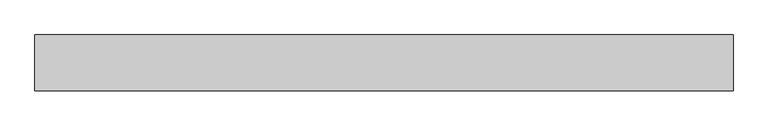
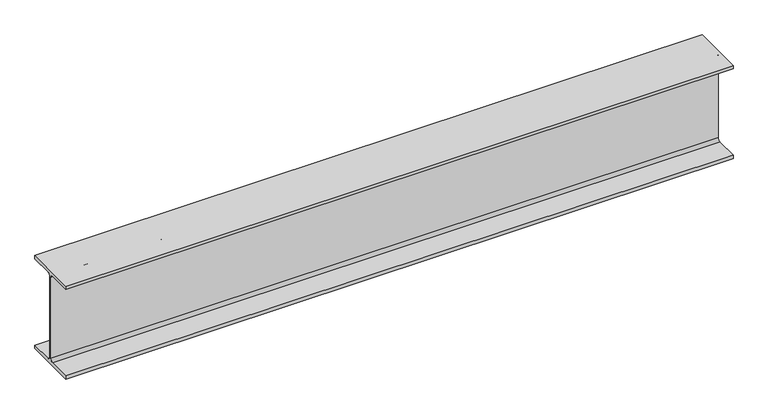
"""IFC4 building model written with IfcOpenShell, lengths in millimetres: beam geometry, Old_Steel Beam_H-KSD3502 : H_SB_ASB_H-194×150x6x9."""

import ifcopenshell
import ifcopenshell.guid

model = None  # the IFC model being written
_history = None  # IfcOwnerHistory: only IFC2X3 demands one
_inside = {}  # id of a spatial element -> (the spatial element, [elements in it])
_under = {}  # id of a project, library or spatial element -> (it, [spatial elements below it])
_declared = {}  # id of a project -> (the project, [libraries it declares])
_typed = {}  # id of a type object -> (the type object, [elements of that type])
_made_of = {}  # id of a material, layer set ... -> (it, [elements and type objects made of it])


def new_model(schema):
    """Start an empty IFC model of exactly this schema.

    Asked for "IFC4X3", IfcOpenShell would pick the latest addendum, in which some entities
    have other attributes; the version numbers below select the first issue.
    IFC2X3 requires an IfcOwnerHistory on every rooted entity: one is made here for all.
    """
    global model, _history
    if schema == "IFC4X3":
        model = ifcopenshell.file(schema_version=(4, 3, 0, 0))
    else:
        model = ifcopenshell.file(schema=schema)
    _inside.clear()
    _under.clear()
    _declared.clear()
    _typed.clear()
    _made_of.clear()
    _history = None
    if model.schema == "IFC2X3":
        org = make("IfcOrganization", Name="unknown")
        user = make(
            "IfcPersonAndOrganization",
            ThePerson=make("IfcPerson", FamilyName="unknown"),
            TheOrganization=org,
        )
        app = make(
            "IfcApplication",
            ApplicationDeveloper=org,
            Version="unknown",
            ApplicationFullName="unknown",
            ApplicationIdentifier="unknown",
        )
        _history = make(
            "IfcOwnerHistory",
            OwningUser=user,
            OwningApplication=app,
            ChangeAction="ADDED",
            CreationDate=0,
        )
    return model


def make(cls, **values):
    """One entity of the class cls with the attributes given. An attribute that is None is left unset."""
    return model.create_entity(
        cls, **{name: value for name, value in values.items() if value is not None}
    )


def rooted(cls, **values):
    """An entity with a GlobalId (a new one), such as an element, a storey or a relation."""
    return make(cls, GlobalId=ifcopenshell.guid.new(), OwnerHistory=_history, **values)


def si_unit(unit_type, name, prefix=None):
    """IfcSIUnit, for example si_unit("LENGTHUNIT", "METRE", prefix="MILLI")."""
    return make("IfcSIUnit", UnitType=unit_type, Prefix=prefix, Name=name)


def assignment(units):
    """IfcUnitAssignment: the units of a project."""
    return None if units is None else make("IfcUnitAssignment", Units=units)


def point(xyz):
    """IfcCartesianPoint."""
    return None if xyz is None else make("IfcCartesianPoint", Coordinates=xyz)


def direction(xyz):
    """IfcDirection."""
    return None if xyz is None else make("IfcDirection", DirectionRatios=xyz)


def frame(location, z_axis=None, x_axis=None):
    """IfcAxis2Placement3D, a coordinate frame: its origin and axes. An axis left out is left unset."""
    return make(
        "IfcAxis2Placement3D",
        Location=point(location),
        Axis=direction(z_axis),
        RefDirection=direction(x_axis),
    )


def frame_2d(location, x_axis=None):
    """IfcAxis2Placement2D, a coordinate frame in the plane: its origin and x axis."""
    return make(
        "IfcAxis2Placement2D", Location=point(location), RefDirection=direction(x_axis)
    )


def origin():
    """The frame at (0, 0, 0) with its axes left unset."""
    return frame((0.0, 0.0, 0.0))


def place(relative_to, where):
    """IfcLocalPlacement: puts the frame where relative to a parent placement (None: the world)."""
    return make(
        "IfcLocalPlacement", PlacementRelTo=relative_to, RelativePlacement=where
    )


def context(
    kind, dimensions, precision=None, world=None, true_north=None, identifier=None
):
    """IfcGeometricRepresentationContext, for example the 3D "Model" context."""
    return make(
        "IfcGeometricRepresentationContext",
        ContextIdentifier=identifier,
        ContextType=kind,
        CoordinateSpaceDimension=dimensions,
        Precision=precision,
        WorldCoordinateSystem=world,
        TrueNorth=true_north,
    )


def project(units=None, contexts=None):
    """IfcProject with its units and contexts."""
    return rooted(
        "IfcProject",
        Name="project",
        RepresentationContexts=contexts,
        UnitsInContext=assignment(units),
    )


def spatial(cls, under=None, at=None, **own):
    """A site, building, storey or space (cls), placed at a placement, below another one or the project."""
    s = rooted(cls, ObjectPlacement=at, **own)
    if under is not None:
        _under.setdefault(under.id(), (under, []))[1].append(s)
    return s


def polyline(points):
    """IfcPolyline through the points."""
    return make("IfcPolyline", Points=[point(p) for p in points])


def circle_curve(where, radius):
    """IfcCircle in the frame where."""
    return make("IfcCircle", Position=where, Radius=radius)


def trimmed(basis, trim1, trim2, sense, master):
    """IfcTrimmedCurve: the piece of a basis curve between two trims."""
    return make(
        "IfcTrimmedCurve",
        BasisCurve=basis,
        Trim1=trim1,
        Trim2=trim2,
        SenseAgreement=sense,
        MasterRepresentation=master,
    )


def segment(curve, same_sense, transition):
    """IfcCompositeCurveSegment."""
    return make(
        "IfcCompositeCurveSegment",
        Transition=transition,
        SameSense=same_sense,
        ParentCurve=curve,
    )


def composite_curve(segments, self_intersect=None):
    """IfcCompositeCurve: segments joined end to end."""
    return make("IfcCompositeCurve", Segments=segments, SelfIntersect=self_intersect)


def outline(outer, holes=None, kind="AREA"):
    """IfcArbitraryClosedProfileDef: a profile drawn as a closed curve; with holes, ...WithVoids."""
    if holes is None:
        return make("IfcArbitraryClosedProfileDef", ProfileType=kind, OuterCurve=outer)
    return make(
        "IfcArbitraryProfileDefWithVoids",
        ProfileType=kind,
        OuterCurve=outer,
        InnerCurves=holes,
    )


def extrude(swept, where, along, depth):
    """IfcExtrudedAreaSolid: the profile swept, set in the frame where, extruded along a direction by depth."""
    return make(
        "IfcExtrudedAreaSolid",
        SweptArea=swept,
        Position=where,
        ExtrudedDirection=direction(along),
        Depth=depth,
    )


def shape(context_of_items, identifier, shape_type, items):
    """IfcShapeRepresentation: the items that make up one representation, for example the "Body"."""
    return make(
        "IfcShapeRepresentation",
        ContextOfItems=context_of_items,
        RepresentationIdentifier=identifier,
        RepresentationType=shape_type,
        Items=items,
    )


def source(mapping_origin, context_of_items, identifier, shape_type, items):
    """IfcRepresentationMap: a shape defined once, which mapped items show again and again."""
    return make(
        "IfcRepresentationMap",
        MappingOrigin=mapping_origin,
        MappedRepresentation=shape(context_of_items, identifier, shape_type, items),
    )


def transform(
    local_origin,
    x_axis=None,
    y_axis=None,
    z_axis=None,
    scale=None,
    scale2=None,
    scale3=None,
    uniform=True,
):
    """IfcCartesianTransformationOperator3D, or its non-uniform kind. x_axis, y_axis, z_axis: its Axis1, 2, 3."""
    if uniform:
        return make(
            "IfcCartesianTransformationOperator3D",
            Axis1=direction(x_axis),
            Axis2=direction(y_axis),
            LocalOrigin=point(local_origin),
            Scale=scale,
            Axis3=direction(z_axis),
        )
    return make(
        "IfcCartesianTransformationOperator3DnonUniform",
        Axis1=direction(x_axis),
        Axis2=direction(y_axis),
        LocalOrigin=point(local_origin),
        Scale=scale,
        Axis3=direction(z_axis),
        Scale2=scale2,
        Scale3=scale3,
    )


def mapped(mapping_source, mapping_target):
    """IfcMappedItem: shows the shape of a source again, moved by a transform."""
    return make(
        "IfcMappedItem", MappingSource=mapping_source, MappingTarget=mapping_target
    )


def made_of(thing, what):
    """Note that an element or type object is made of a material, layer set ...; save() writes the relation."""
    if what is not None:
        _made_of.setdefault(what.id(), (what, []))[1].append(thing)
    return thing


def element(
    cls,
    number,
    at=None,
    inside=None,
    cuts=None,
    type_object=None,
    material=None,
    context=None,
    identifier="Body",
    shape_type=None,
    held_by="IfcProductDefinitionShape",
    body=None,
    shapes=None,
    **own,
):
    """One element of the class cls, such as IfcWall. Its Tag is "e" and its number.

    at: its placement. inside: the storey or other place that contains it. cuts: it is an
    opening in that element (IfcRelVoidsElement). A single representation is given by context,
    identifier, shape_type and body (its items); several are given by shapes. held_by: the class
    of the entity that holds the representations. save() writes the other relations.
    """
    e = rooted(cls, Tag="e%d" % number, ObjectPlacement=at, **own)
    if body is not None:
        shapes = [shape(context, identifier, shape_type, body)]
    if shapes is not None:
        e.Representation = make(held_by, Representations=shapes)
    if inside is not None:
        _inside.setdefault(inside.id(), (inside, []))[1].append(e)
    if cuts is not None:
        rooted(
            "IfcRelVoidsElement", RelatingBuildingElement=cuts, RelatedOpeningElement=e
        )
    if type_object is not None:
        _typed.setdefault(type_object.id(), (type_object, []))[1].append(e)
    return made_of(e, material)


def aggregate(whole, parts):
    """IfcRelAggregates: a whole, such as a stair, and the parts it consists of."""
    return rooted("IfcRelAggregates", RelatingObject=whole, RelatedObjects=parts)


def save(model, path):
    """Write the relations noted so far, then the file.

    IfcRelAggregates (storeys below a building ...), IfcRelContainedInSpatialStructure (elements
    in a storey), IfcRelDefinesByType, IfcRelAssociatesMaterial and IfcRelDeclares: one each for
    every whole, place, type object, material and project.
    """
    for whole, parts in _under.values():
        aggregate(whole, parts)
    for where, things in _inside.values():
        rooted(
            "IfcRelContainedInSpatialStructure",
            RelatedElements=things,
            RelatingStructure=where,
        )
    for kind, things in _typed.values():
        rooted("IfcRelDefinesByType", RelatedObjects=things, RelatingType=kind)
    for what, things in _made_of.values():
        rooted("IfcRelAssociatesMaterial", RelatedObjects=things, RelatingMaterial=what)
    for by, libraries in _declared.values():
        rooted("IfcRelDeclares", RelatingContext=by, RelatedDefinitions=libraries)
    model.write(path)


def beam_ff7b883b(model_context):
    return source(origin(), model_context, "Body", "SweptSolid", [
        extrude(outline(composite_curve([segment(polyline([(-82.5, -141.5), (-11.9, -141.5)]), True, "CONTINUOUS"), segment(trimmed(circle_curve(frame_2d((-11.9, -132.6)), 8.9), [point((-11.9, -141.5))], [point((-3.0, -132.6))], True, "CARTESIAN"), True, "CONTINUOUS"), segment(polyline([(-3.0, -132.6), (-3.0, 132.6)]), True, "CONTINUOUS"), segment(trimmed(circle_curve(frame_2d((-11.9, 132.6)), 8.9), [point((-3.0, 132.6))], [point((-11.9, 141.5))], True, "CARTESIAN"), True, "CONTINUOUS"), segment(polyline([(-11.9, 141.5), (-82.5, 141.5), (-82.5, 151.7), (82.5, 151.7), (82.5, 141.5), (11.9, 141.5)]), True, "CONTINUOUS"), segment(trimmed(circle_curve(frame_2d((11.9, 132.6)), 8.9), [point((11.9, 141.5))], [point((3.0, 132.6))], True, "CARTESIAN"), True, "CONTINUOUS"), segment(polyline([(3.0, 132.6), (3.0, -132.6)]), True, "CONTINUOUS"), segment(trimmed(circle_curve(frame_2d((11.9, -132.6)), 8.9), [point((3.0, -132.6))], [point((11.9, -141.5))], True, "CARTESIAN"), True, "CONTINUOUS"), segment(polyline([(11.9, -141.5), (82.5, -141.5), (82.5, -151.7), (-82.5, -151.7), (-82.5, -141.5)]), True, "CONTINUOUS")], self_intersect=False)), frame((-1171.2564634, 0.0, 0.0), z_axis=(1.0, 0.0, 0.0), x_axis=(0.0, 1.0, 0.0)), (0.0, 0.0, 1.0), 2060.1030758),
    ])


if __name__ == "__main__":
    model = new_model("IFC4")
    model_context = context("Model", 3, world=origin())
    ifc_project = project(units=[si_unit("LENGTHUNIT", "METRE", prefix="MILLI")], contexts=[model_context])
    site = spatial("IfcSite", under=ifc_project)
    building = spatial("IfcBuilding", under=site)
    placement = place(None, origin())
    beam_shape = beam_ff7b883b(model_context)
    element("IfcBeam", 1, ObjectType="Old_Steel Beam_H-KSD3502 : H_SB_ASB_H-194×150x6x9", at=placement, inside=building, context=model_context, shape_type="MappedRepresentation", body=[
        mapped(beam_shape, transform((0.0, 0.0, 0.0), x_axis=(1.0, 0.0, 0.0), y_axis=(0.0, 1.0, 0.0), z_axis=(0.0, 0.0, 1.0))),
    ])
    save(model, "model.ifc")

# Revit data of these elements
# Type "Old_Steel Beam_H-KSD3502 : H_SB_ASB_H-194×150x6x9"
#   Width = 15.0 cm
#   Web Thickness = 0.6 cm
#   Web Fillet = 1.3 cm
#   Warping Constant = 43316.0 cm⁶
#   Torsional Moment of Inertia = 8.622 cm⁴
#   Torsional Modulus = 1.0 cm³
#   Section Area = 39.01 cm²
#   Plastic Modulus weak axis = 104.0 cm³
#   Plastic Modulus strong axis = 309.0 cm³
#   Perimeter = 0.95 m²/m
#   Nominal Weight = 30.60 kgf/m
#   Moment of Inertia weak axis = 507.00 cm⁴
#   Moment of Inertia strong axis = 2690.00 cm⁴
#   Height = 19.4 cm
#   Flange Thickness = 0.9 cm
#   Elastic Modulus weak axis = 67.6 cm³
#   Elastic Modulus strong axis = 277.0 cm³
#   Centroid Vertical = 9.7 cm
#   Centroid Horizontal = 7.5 cm
#   Length [instance default] = 1.5240 m
#   Structural Material [instance default] = Steel, 45-345
#   Assembly Code = ""
# Element 1 (IfcBeam, "Old_Steel Beam_H-KSD3502 : H_SB_ASB_H-194×150x6x9")
#   Structural Material = none
# Materials
#   "Steel, 45-345": class "Metal", colour RGB 189 187 185, transparency 0, Description = "Steel 345 MPa", Cost = 0
